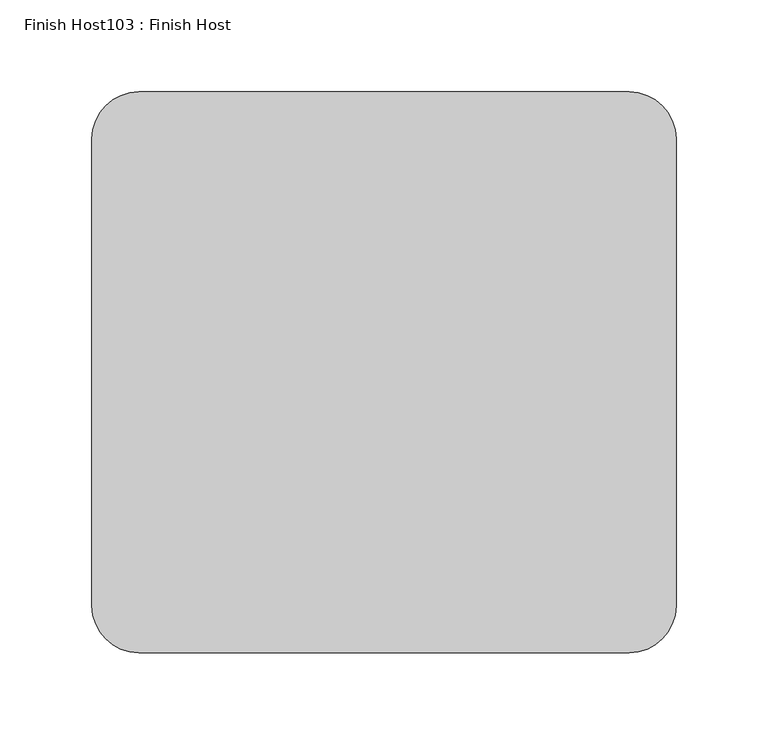
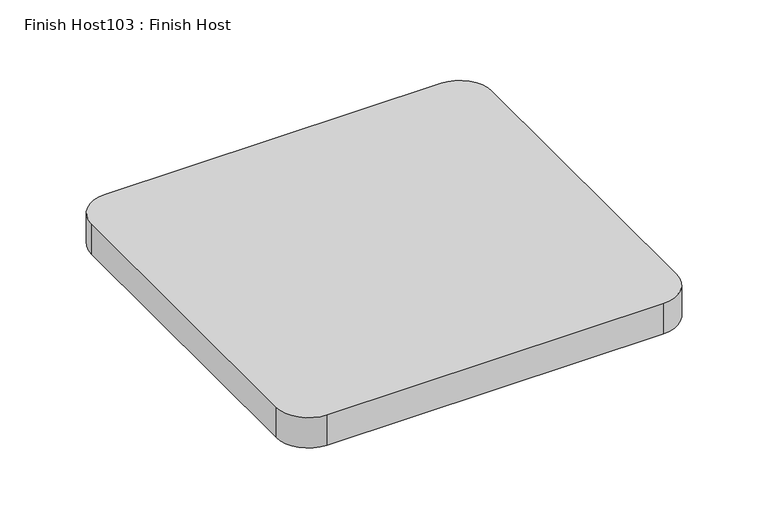
"""IFC4 building model written with IfcOpenShell, lengths in millimetres: proxy geometry, Finish Host103 : Finish Host."""

from ifc_helpers import new_model, si_unit, point, frame_2d, origin, origin_with_axes, place, context, project, spatial, polyline, circle_curve, trimmed, segment, composite_curve, outline, extrude, source, transform, mapped, element, save


def finish_host103_finish_host_2782fa5f(model_context):
    return source(origin(), model_context, "Body", "SweptSolid", [
        extrude(outline(composite_curve([segment(polyline([(-47.8842816, 4229.4760864), (-47.8842816, 4483.4760864)]), True, "CONTINUOUS"), segment(trimmed(circle_curve(frame_2d((-22.4842816, 4483.4760864)), 25.4), [point((-47.8842816, 4483.4760864))], [point((-22.4842816, 4508.8760864))], False, "CARTESIAN"), True, "CONTINUOUS"), segment(polyline([(-22.4842816, 4508.8760864), (244.2157184, 4508.8760864)]), True, "CONTINUOUS"), segment(trimmed(circle_curve(frame_2d((244.2157184, 4483.4760864)), 25.4), [point((244.2157184, 4508.8760864))], [point((269.6157184, 4483.4760864))], False, "CARTESIAN"), True, "CONTINUOUS"), segment(polyline([(269.6157184, 4483.4760864), (269.6157184, 4229.4760864)]), True, "CONTINUOUS"), segment(trimmed(circle_curve(frame_2d((244.2157184, 4229.4760864)), 25.4), [point((269.6157184, 4229.4760864))], [point((244.2157184, 4204.0760864))], False, "CARTESIAN"), True, "CONTINUOUS"), segment(polyline([(244.2157184, 4204.0760864), (-22.4842816, 4204.0760864)]), True, "CONTINUOUS"), segment(trimmed(circle_curve(frame_2d((-22.4842816, 4229.4760864)), 25.4), [point((-22.4842816, 4204.0760864))], [point((-47.8842816, 4229.4760864))], False, "CARTESIAN"), True, "CONTINUOUS")], self_intersect=False)), origin_with_axes(), (0.0, 0.0, 1.0), 25.4),
    ])


if __name__ == "__main__":
    model = new_model("IFC4")
    model_context = context("Model", 3, world=origin())
    ifc_project = project(units=[si_unit("LENGTHUNIT", "METRE", prefix="MILLI")], contexts=[model_context])
    site = spatial("IfcSite", under=ifc_project)
    building = spatial("IfcBuilding", under=site)
    placement = place(None, origin())
    finish_host103_finish_host_shape = finish_host103_finish_host_2782fa5f(model_context)
    element("IfcBuildingElementProxy", 1, Name="Finish Host103 : Finish Host", ObjectType="Finish Host103 : Finish Host", at=placement, inside=building, context=model_context, shape_type="MappedRepresentation", body=[
        mapped(finish_host103_finish_host_shape, transform((0.0, 0.0, 0.0), x_axis=(1.0, 0.0, 0.0), y_axis=(0.0, 1.0, 0.0), z_axis=(0.0, 0.0, 1.0))),
    ])
    save(model, "model.ifc")

# Revit data of these elements
# Type "Finish Host103 : Finish Host"
#   Countertop Material = Fabric - Teknion - P109 - Percept - Methodic
# Element 1 (IfcBuildingElementProxy, "Finish Host103 : Finish Host")
#   Materials on its faces: "Fabric - Teknion - P109 - Percept - Methodic"
# Materials
#   "Fabric - Teknion - P109 - Percept - Methodic": class "Generic", colour RGB 51 46 43, transparency 0, Model = "P109", Manufacturer = "Teknion Textiles", URL = "http://www.tekniontextiles.ca/", Description = "Methodic Percept", Cost = 0
